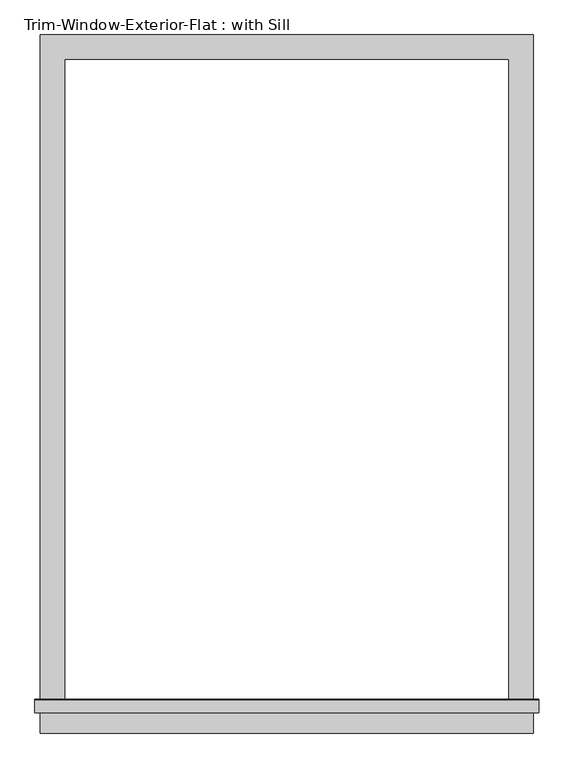
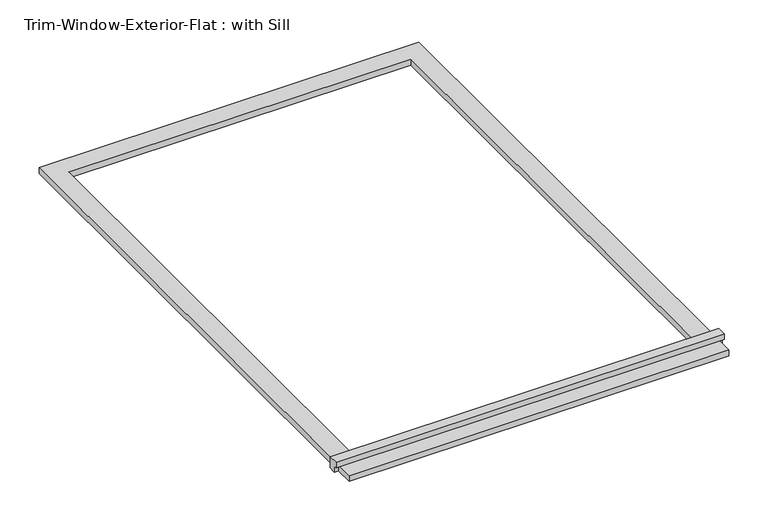
"""IFC4 building model written with IfcOpenShell, lengths in millimetres: proxy geometry, Trim-Window-Exterior-Flat : with Sill."""

from ifc_helpers import new_model, si_unit, frame, origin, origin_with_axes, place, context, project, spatial, polyline, outline, extrude, source, transform, mapped, element, save


def trim_window_exterior_flat_with_sill_7e0c1154(model_context):
    return source(origin(), model_context, "Body", "SweptSolid", [
        extrude(outline(polyline([(577.85, -1520.7823709), (577.85, -1577.9323709), (-577.85, -1577.9323709), (-577.85, -1520.7823709), (577.85, -1520.7823709)])), origin_with_axes(), (0.0, 0.0, 1.0), 19.05),
        extrude(outline(polyline([(-1530.35, 38.1), (-1501.0580645, 38.1), (-1498.6, 19.05), (-1498.6, 0.0), (-1520.7823709, 0.0), (-1520.7823709, 19.05), (-1530.35, 19.05), (-1530.35, 38.1)])), frame((-590.55, 0.0, 0.0), z_axis=(1.0, 0.0, 0.0), x_axis=(0.0, 1.0, 0.0)), (0.0, 0.0, 1.0), 1181.1),
        extrude(outline(polyline([(-577.85, 57.15), (577.85, 57.15), (577.85, -1498.6), (520.7, -1498.6), (520.7, 0.0), (-520.7, 0.0), (-520.7, -1498.6), (-577.85, -1498.6), (-577.85, 57.15)])), origin_with_axes(), (0.0, 0.0, 1.0), 19.05),
    ])


if __name__ == "__main__":
    model = new_model("IFC4")
    model_context = context("Model", 3, world=origin())
    ifc_project = project(units=[si_unit("LENGTHUNIT", "METRE", prefix="MILLI")], contexts=[model_context])
    site = spatial("IfcSite", under=ifc_project)
    building = spatial("IfcBuilding", under=site)
    placement = place(None, origin())
    trim_window_exterior_flat_with_sill_shape = trim_window_exterior_flat_with_sill_7e0c1154(model_context)
    element("IfcBuildingElementProxy", 1, Name="Trim-Window-Exterior-Flat : with Sill", ObjectType="Trim-Window-Exterior-Flat : with Sill", at=placement, inside=building, context=model_context, shape_type="MappedRepresentation", body=[
        mapped(trim_window_exterior_flat_with_sill_shape, transform((0.0, 0.0, 0.0), x_axis=(1.0, 0.0, 0.0), y_axis=(0.0, 1.0, 0.0), z_axis=(0.0, 0.0, 1.0))),
    ])
    save(model, "model.ifc")

# Revit data of these elements
# Type "Trim-Window-Exterior-Flat : with Sill"
#   Trim Width = 0' - 2 1/4"
#   Trim Thickness_Picture Frame = 0' - 1 1/4"
#   Trim Thickness_with Sill = 0' - 0 3/4"
#   Sill Thickness = 0' - 1 1/4"
#   Opening Width [instance default] = 2' - 0"
#   Opening Height [instance default] = 3' - 0"
#   Default Elevation = 4' - 0"
#   Sill = yes
#   Picture Frame = no
#   Trim Material [instance default] = none
# Element 1 (IfcBuildingElementProxy, "Trim-Window-Exterior-Flat : with Sill")
#   Opening Width = 3' - 5"
#   Opening Height = 4' - 11"
#   Trim Material = 1X WOOD COMPOSITE TRIM
#   Materials on its faces: "1X WOOD COMPOSITE TRIM"
# Materials
#   "1X WOOD COMPOSITE TRIM": class "Generic", colour RGB 88 61 61, transparency 0, Cost = 0
